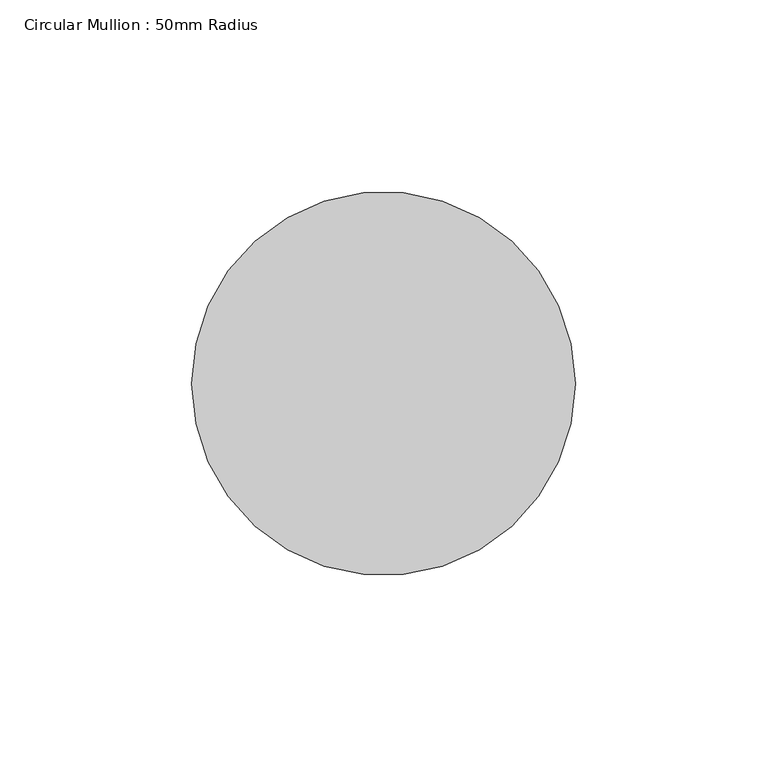
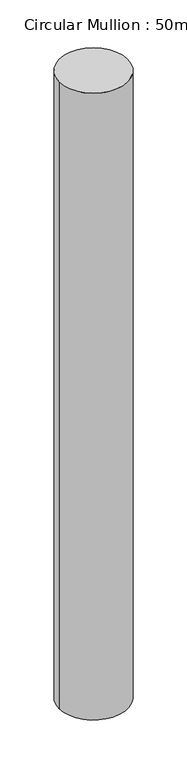
"""IFC4 building model written with IfcOpenShell, lengths in millimetres: member geometry, Circular Mullion : 50mm Radius."""

from ifc_helpers import new_model, si_unit, point, frame, origin, origin_2d, place, context, project, spatial, circle_curve, trimmed, segment, composite_curve, outline, extrude, source, transform, mapped, element, save


def circular_mullion_50mm_radius_2b522084(model_context):
    return source(origin(), model_context, "Body", "SweptSolid", [
        extrude(outline(composite_curve([segment(trimmed(circle_curve(origin_2d(), 50.0), [point((50.0, 0.0))], [point((-50.0, 0.0))], False, "CARTESIAN"), True, "CONTINUOUS"), segment(trimmed(circle_curve(origin_2d(), 50.0), [point((-50.0, 0.0))], [point((50.0, 0.0))], False, "CARTESIAN"), True, "CONTINUOUS")], self_intersect=False)), frame((0.0, 0.0, -966.6726449), z_axis=(0.0, 0.0, 1.0), x_axis=(1.0, 0.0, 0.0)), (0.0, 0.0, 1.0), 966.6726449),
    ])


if __name__ == "__main__":
    model = new_model("IFC4")
    model_context = context("Model", 3, world=origin())
    ifc_project = project(units=[si_unit("LENGTHUNIT", "METRE", prefix="MILLI")], contexts=[model_context])
    site = spatial("IfcSite", under=ifc_project)
    building = spatial("IfcBuilding", under=site)
    placement = place(None, origin())
    circular_mullion_50mm_radius_shape = circular_mullion_50mm_radius_2b522084(model_context)
    element("IfcMember", 1, ObjectType="Circular Mullion : 50mm Radius", at=placement, inside=building, context=model_context, shape_type="MappedRepresentation", body=[
        mapped(circular_mullion_50mm_radius_shape, transform((0.0, 0.0, 0.0), x_axis=(1.0, 0.0, 0.0), y_axis=(0.0, 1.0, 0.0), z_axis=(0.0, 0.0, 1.0))),
    ])
    save(model, "model.ifc")

# Revit data of these elements
# Type "Circular Mullion : 50mm Radius"
#   built-in parameter 1007350 = 0.164042 (stored number, unit not read)
# Element 1 (IfcMember, "Circular Mullion : 50mm Radius")
#   Materials on its faces: "Aluminium"
# Materials
#   "Aluminium": class "Metal", colour RGB 247 247 247, transparency 0, Description = "Aluminium 6061", Cost = 0
